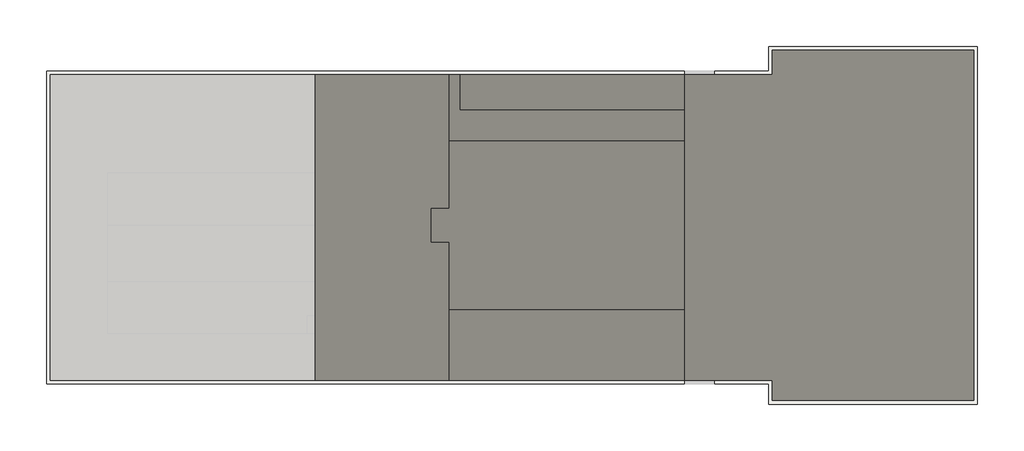
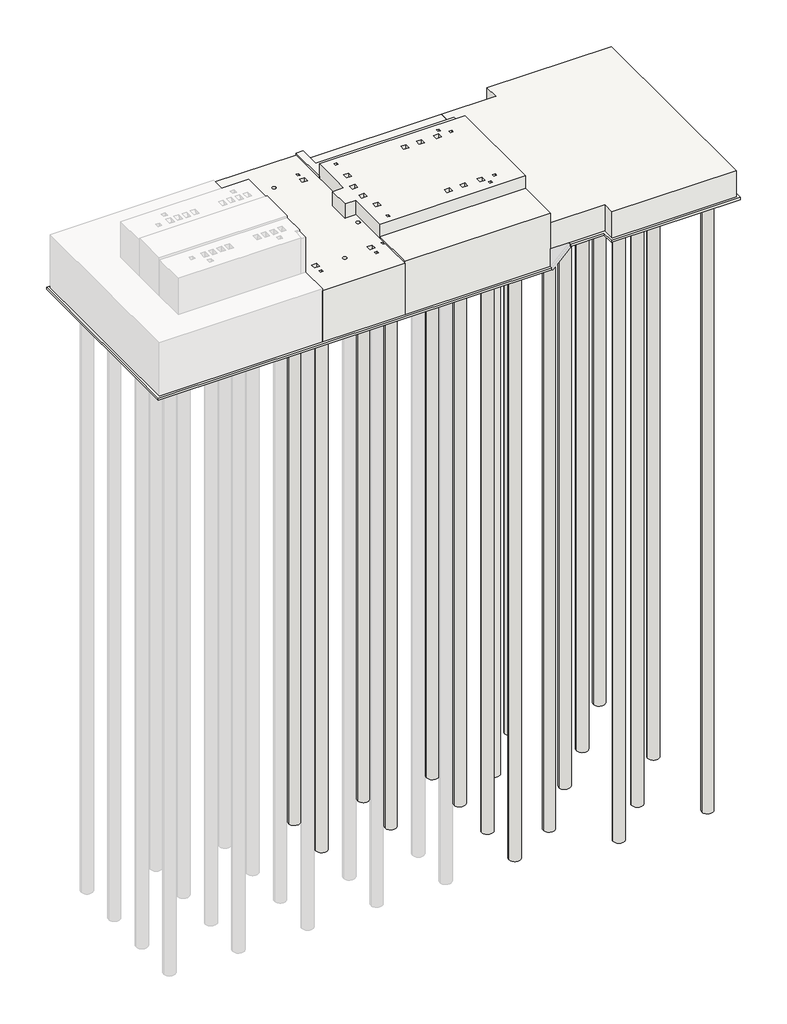
# One storey, part 2 of 2: 25 slabs.
# Revit data of these elements (continued)
# Type "H_SF_AR_B01_EQ FDN_Bitumen_Mat T2440"
#   Type Comments = "구조_콘크리트"
#   Type Mark = "MF00"
#   Layers, outside or top first: 2440 mm "Concrete_f'c=24MPa(Cylender)" (function 1)
# Type "H_SF_AR_B01_EQ FDN_Bitumen_Mat T2000"
#   Type Comments = "구조_콘크리트"
#   Type Mark = "MF00"
#   Layers, outside or top first: 2000 mm "Concrete_f'c=24MPa(Cylender)" (function 1)
# Type "H_SF_AR_B01_EQ FDN_Bitumen_Mat T3010"
#   Type Comments = "구조_콘크리트"
#   Type Mark = "MF00"
#   Layers, outside or top first: 3010 mm "Concrete_f'c=24MPa(Cylender)" (function 1)
# Type "H_SF_AR_B01_EQ FDN_Bitumen_Mat T2350"
#   Type Comments = "구조_콘크리트"
#   Type Mark = "MF00"
#   Layers, outside or top first: 2350 mm "Concrete_f'c=24MPa(Cylender)" (function 1)
# Type "H_SF_AR_B01_EQ FDN_Bitumen_Mat T1200"
#   Type Comments = "구조_콘크리트"
#   Type Mark = "MF00"
#   Layers, outside or top first: 1200 mm "Concrete_f'c=24MPa(Cylender)" (function 1)
# Type "H_SF_AR_S18_Lean_T100"
#   Type Comments = "구조_콘크리트"
#   Layers, outside or top first: 100 mm "Concrete_Lean_f'c=14MPa(Cylender)" (function 1)
# Type "PILE : H_SF_AR_S19_PHC Pile_Hammering_D500_L27.4"
#   Type Comments = "CV-UG"
#   Assembly Code = "A1020120"
#   반지름 = 250 mm
#   최소 내포 = 100 mm
#   Diameter = 500 mm
#   Depth = 27400 mm
#   Structural Material [instance default] = none
# Type "PILE : H_SF_AR_S19_PHC Pile_Hammering_D500_L28.2"
#   Type Comments = "CV-UG"
#   Assembly Code = "A1020120"
#   반지름 = 250 mm
#   최소 내포 = 100 mm
#   Diameter = 500 mm
#   Depth = 28200 mm
#   Structural Material [instance default] = none
# Element 1 (IfcSlab, "H_SF_AR_B01_EQ FDN_Bitumen_Mat T2440")
#   Comments = ""
#   Height Offset From Level = 2440 mm
#   built-in parameter 1001954 = 1
#   Phase Created = New Construction
#   Materials on its faces: "Concrete_f'c=24MPa(Cylender)"
# Element 2 (IfcSlab, "H_SF_AR_B01_EQ FDN_Bitumen_Mat T2000")
#   Comments = ""
#   Height Offset From Level = 2000 mm
#   built-in parameter 1001954 = 1
#   Phase Created = New Construction
#   Materials on its faces: "Concrete_f'c=24MPa(Cylender)"
# Element 3 (IfcSlab, "H_SF_AR_B01_EQ FDN_Bitumen_Mat T3010")
#   Comments = ""
#   built-in parameter 1001955 = -1.5708 (stored number, unit not read)
#   Height Offset From Level = 3010 mm
#   built-in parameter 1001954 = 1
#   Phase Created = New Construction
#   Materials on its faces: "Concrete_f'c=24MPa(Cylender)"
# Element 4 (IfcSlab, "H_SF_AR_B01_EQ FDN_Bitumen_Mat T2350")
#   Comments = ""
#   Height Offset From Level = 2350 mm
#   built-in parameter 1001954 = 1
#   Phase Created = New Construction
#   Materials on its faces: "Concrete_f'c=24MPa(Cylender)"
# Element 5 (IfcSlab, "H_SF_AR_B01_EQ FDN_Bitumen_Mat T1200")
#   Comments = ""
#   Height Offset From Level = 2000 mm
#   built-in parameter 1001954 = 1
#   Phase Created = New Construction
#   Materials on its faces: "Concrete_f'c=24MPa(Cylender)"
# Element 6 (IfcSlab, "H_SF_AR_S18_Lean_T100")
#   Comments = ""
#   Height Offset From Level = 0 mm
#   built-in parameter 1001954 = 1
#   Phase Created = New Construction
#   Materials on its faces: "Concrete_Lean_f'c=14MPa(Cylender)"
# Element 7 (IfcSlab, "H_SF_AR_S18_Lean_T100")
#   Comments = ""
#   Height Offset From Level = 800 mm
#   built-in parameter 1001954 = 1
#   Phase Created = New Construction
#   Materials on its faces: "Concrete_Lean_f'c=14MPa(Cylender)"
# Element 8 (IfcSlab, "PILE : H_SF_AR_S19_PHC Pile_Hammering_D500_L27.4")
#   Mark = "013"
#   Structural Material = Concrete_f'c=28MPa(Cylender)
#   Phase Created = New Construction
#   Materials on its faces: "Concrete_f'c=28MPa(Cylender)"
# Element 9 (IfcSlab, "PILE : H_SF_AR_S19_PHC Pile_Hammering_D500_L27.4")
#   Mark = "014"
#   Structural Material = Concrete_f'c=28MPa(Cylender)
#   Phase Created = New Construction
#   Materials on its faces: "Concrete_f'c=28MPa(Cylender)"
# Element 10 (IfcSlab, "PILE : H_SF_AR_S19_PHC Pile_Hammering_D500_L27.4")
#   Mark = "018"
#   Structural Material = Concrete_f'c=28MPa(Cylender)
#   Phase Created = New Construction
#   Materials on its faces: "Concrete_f'c=28MPa(Cylender)"
# Element 11 (IfcSlab, "PILE : H_SF_AR_S19_PHC Pile_Hammering_D500_L27.4")
#   Mark = "017"
#   Structural Material = Concrete_f'c=28MPa(Cylender)
#   Phase Created = New Construction
#   Materials on its faces: "Concrete_f'c=28MPa(Cylender)"
# Element 12 (IfcSlab, "PILE : H_SF_AR_S19_PHC Pile_Hammering_D500_L27.4")
#   Mark = "021"
#   Structural Material = Concrete_f'c=28MPa(Cylender)
#   Phase Created = New Construction
#   Materials on its faces: "Concrete_f'c=28MPa(Cylender)"
# Element 13 (IfcSlab, "PILE : H_SF_AR_S19_PHC Pile_Hammering_D500_L27.4")
#   Mark = "022"
#   Structural Material = Concrete_f'c=28MPa(Cylender)
#   Phase Created = New Construction
#   Materials on its faces: "Concrete_f'c=28MPa(Cylender)"
# Element 14 (IfcSlab, "PILE : H_SF_AR_S19_PHC Pile_Hammering_D500_L27.4")
#   Mark = "023"
#   Structural Material = Concrete_f'c=28MPa(Cylender)
#   Phase Created = New Construction
#   Materials on its faces: "Concrete_f'c=28MPa(Cylender)"
# Element 15 (IfcSlab, "PILE : H_SF_AR_S19_PHC Pile_Hammering_D500_L27.4")
#   Mark = "024"
#   Structural Material = Concrete_f'c=28MPa(Cylender)
#   Phase Created = New Construction
#   Materials on its faces: "Concrete_f'c=28MPa(Cylender)"
# Element 16 (IfcSlab, "PILE : H_SF_AR_S19_PHC Pile_Hammering_D500_L28.2")
#   Mark = "025"
#   Structural Material = Concrete_f'c=28MPa(Cylender)
#   Phase Created = New Construction
#   Materials on its faces: "Concrete_f'c=28MPa(Cylender)"
# Element 17 (IfcSlab, "PILE : H_SF_AR_S19_PHC Pile_Hammering_D500_L28.2")
#   Mark = "026"
#   Structural Material = Concrete_f'c=28MPa(Cylender)
#   Phase Created = New Construction
#   Materials on its faces: "Concrete_f'c=28MPa(Cylender)"
# Element 18 (IfcSlab, "PILE : H_SF_AR_S19_PHC Pile_Hammering_D500_L28.2")
#   Mark = "027"
#   Structural Material = Concrete_f'c=28MPa(Cylender)
#   Phase Created = New Construction
#   Materials on its faces: "Concrete_f'c=28MPa(Cylender)"
# Element 19 (IfcSlab, "PILE : H_SF_AR_S19_PHC Pile_Hammering_D500_L28.2")
#   Mark = "032"
#   Structural Material = Concrete_f'c=28MPa(Cylender)
#   Phase Created = New Construction
#   Materials on its faces: "Concrete_f'c=28MPa(Cylender)"
# Element 20 (IfcSlab, "PILE : H_SF_AR_S19_PHC Pile_Hammering_D500_L28.2")
#   Mark = "028"
#   Structural Material = Concrete_f'c=28MPa(Cylender)
#   Phase Created = New Construction
#   Materials on its faces: "Concrete_f'c=28MPa(Cylender)"
# Element 21 (IfcSlab, "PILE : H_SF_AR_S19_PHC Pile_Hammering_D500_L28.2")
#   Mark = "031"
#   Structural Material = Concrete_f'c=28MPa(Cylender)
#   Phase Created = New Construction
#   Materials on its faces: "Concrete_f'c=28MPa(Cylender)"
# Element 22 (IfcSlab, "PILE : H_SF_AR_S19_PHC Pile_Hammering_D500_L28.2")
#   Mark = "029"
#   Structural Material = Concrete_f'c=28MPa(Cylender)
#   Phase Created = New Construction
#   Materials on its faces: "Concrete_f'c=28MPa(Cylender)"
# Element 23 (IfcSlab, "PILE : H_SF_AR_S19_PHC Pile_Hammering_D500_L28.2")
#   Mark = "034"
#   Structural Material = Concrete_f'c=28MPa(Cylender)
#   Phase Created = New Construction
#   Materials on its faces: "Concrete_f'c=28MPa(Cylender)"
# Element 24 (IfcSlab, "PILE : H_SF_AR_S19_PHC Pile_Hammering_D500_L28.2")
#   Mark = "033"
#   Structural Material = Concrete_f'c=28MPa(Cylender)
#   Phase Created = New Construction
#   Materials on its faces: "Concrete_f'c=28MPa(Cylender)"
# Element 25 (IfcSlab, "PILE : H_SF_AR_S19_PHC Pile_Hammering_D500_L28.2")
#   Mark = "030"
#   Structural Material = Concrete_f'c=28MPa(Cylender)
#   Phase Created = New Construction
#   Materials on its faces: "Concrete_f'c=28MPa(Cylender)"
# Materials
#   "Concrete_f'c=24MPa(Cylender)": class "Concrete", colour RGB 176 176 176, transparency 0, Description = "EPOXY PAINT\rON STEEL TROWEL FINISH", Cost = 0, Image = Concrete.Cast-In-Place.Flat.Polished.Grey.jpg
#   "Concrete_Lean_f'c=14MPa(Cylender)": class "Concrete", colour RGB 177 177 177, transparency 0, Description = "Reinf. Conc.", Cost = 0
#   "Concrete_f'c=28MPa(Cylender)": class "Concrete", colour RGB 176 176 176, transparency 0, Description = "Reinf. Conc.", Cost = 0, Image = Concrete.Cast-In-Place.Flat.Polished.Grey.jpg
